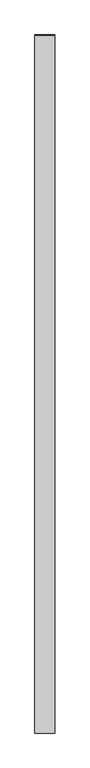
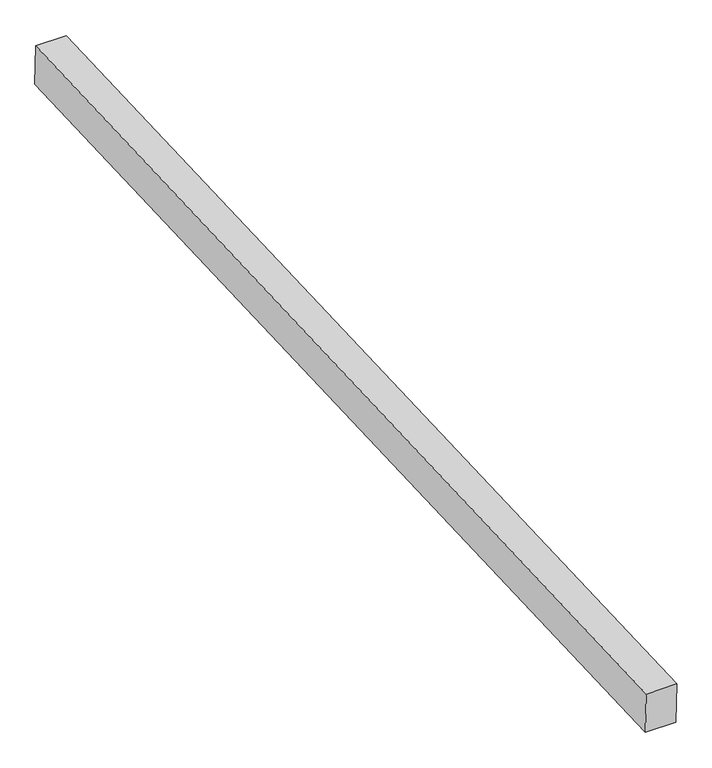
"""IFC4 building model written with IfcOpenShell, lengths in millimetres: proxy geometry, Generic Models 7:Generic Models 1:8:Generic Models 1:8 : Generic Models 7:Generic Models 1:337419:29 : Generic Models 7:Generic Models 1:8:Generic Models 1:8 : Generic Models 7:Generic Models 1:337419:315935."""

from ifc_helpers import new_model, si_unit, frame, origin, place, context, project, spatial, polyline, outline, extrude, source, transform, mapped, element, save


def generic_models_703c046f(model_context):
    return source(origin(), model_context, "Body", "SweptSolid", [
        extrude(outline(polyline([(-569809.5331551, 8697.9424054), (-564936.6102609, 8900.9808594), (-564929.0433392, 8710.6308549), (-569801.6025364, 8507.607555), (-569809.5331551, 8697.9424054)])), frame((588762.8617243, 0.0, 0.0), z_axis=(1.0, 0.0, 0.0), x_axis=(0.0, 1.0, 0.0)), (0.0, 0.0, 1.0), 139.7),
    ])


if __name__ == "__main__":
    model = new_model("IFC4")
    model_context = context("Model", 3, world=origin())
    ifc_project = project(units=[si_unit("LENGTHUNIT", "METRE", prefix="MILLI")], contexts=[model_context])
    site = spatial("IfcSite", under=ifc_project)
    building = spatial("IfcBuilding", under=site)
    placement = place(None, origin())
    generic_models_shape = generic_models_703c046f(model_context)
    element("IfcBuildingElementProxy", 1, Name="Generic Models 7:Generic Models 1:8:Generic Models 1:8 : Generic Models 7:Generic Models 1:337419:29 : Generic Models 7:Generic Models 1:8:Generic Models 1:8 : Generic Models 7:Generic Models 1:337419:315935", ObjectType="Generic Models 7:Generic Models 1:8:Generic Models 1:8 : Generic Models 7:Generic Models 1:337419:29 : Generic Models 7:Generic Models 1:8:Generic Models 1:8 : Generic Models 7:Generic Models 1:337419:315935", at=placement, inside=building, context=model_context, shape_type="MappedRepresentation", body=[
        mapped(generic_models_shape, transform((0.0, 0.0, 0.0), x_axis=(1.0, 0.0, 0.0), y_axis=(0.0, 1.0, 0.0), z_axis=(0.0, 0.0, 1.0))),
    ])
    save(model, "model.ifc")

# Revit data of these elements
# Type "Generic Models 7:Generic Models 1:8:Generic Models 1:8 : Generic Models 7:Generic Models 1:337419:29 : Generic Models 7:Generic Models 1:8:Generic Models 1:8 : Generic Models 7:Generic Models 1:337419:315935"
#   NameOverride = "Generic Models 7:Generic Models 1:8:Generic Models 1:8 : Generic Models 7:Generic Models 1:337419:315935"
#   ObjectTypeOverride = "Generic Models 1:8 : Generic Models 7:Generic Models 1:337419"
#   Reference = "Generic Models 1"
#   Tag = "315935"
# Element 1 (IfcBuildingElementProxy, "Generic Models 7:Generic Models 1:8:Generic Models 1:8 : Generic Models 7:Generic Models 1:337419:29 : Generic Models 7:Generic Models 1:8:Generic Models 1:8 : Generic Models 7:Generic Models 1:337419:315935")
#   Materials on its faces: "5 1/2\" X 7 1/2\" EXTERIOR GRADE GLULAM BEAMS"
# Materials
#   "5 1/2\" X 7 1/2\" EXTERIOR GRADE GLULAM BEAMS": class "Wood", colour RGB 183 134 68, transparency 0, Keynote = "M06181300.01", Description = "Pinus Echinata", Cost = 0
